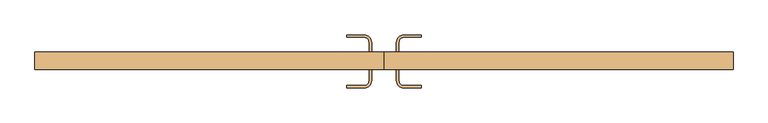
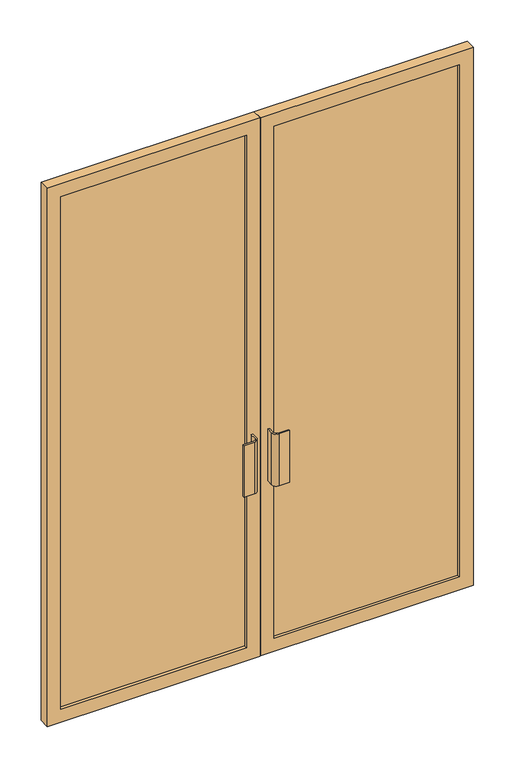
"""IFC4 building model written with IfcOpenShell, lengths in millimetres: door geometry, Porta-Parede-Cortina-Frente de loja-Dupla : Porta-Parede-Cortina-Frente de loja-Dupla."""

from ifc_helpers import new_model, si_unit, point, frame, frame_2d, origin, place, context, project, spatial, polyline, circle_curve, trimmed, segment, composite_curve, outline, extrude, source, transform, mapped, element, save


def door_024b7173(model_context):
    return source(origin(), model_context, "Body", "SweptSolid", [
        extrude(outline(polyline([(2375.0, 0.8168501), (0.0, 0.8168501), (0.0, 890.0), (2375.0, 890.0), (2375.0, 0.8168501)]), holes=[polyline([(2317.85, 57.9668501), (2317.85, 832.85), (57.15, 832.85), (57.15, 57.9668501), (2317.85, 57.9668501)])]), frame((0.0, 15.55, 0.0), z_axis=(0.0, 1.0, 0.0), x_axis=(0.0, 0.0, 1.0)), (0.0, 0.0, 1.0), 44.45),
        extrude(outline(polyline([(2375.0, -0.7706499), (2375.0, -890.0), (0.0, -890.0), (0.0, -0.7706499), (2375.0, -0.7706499)]), holes=[polyline([(2317.85, -832.85), (2317.85, -57.9206499), (57.15, -57.9206499), (57.15, -832.85), (2317.85, -832.85)])]), frame((0.0, 15.55, 0.0), z_axis=(0.0, 1.0, 0.0), x_axis=(0.0, 0.0, 1.0)), (0.0, 0.0, 1.0), 44.45),
        extrude(outline(polyline([(832.85, 28.25), (57.9668501, 28.25), (57.9668501, 47.3), (832.85, 47.3), (832.85, 28.25)])), frame((0.0, 0.0, 57.15), z_axis=(0.0, 0.0, 1.0), x_axis=(1.0, 0.0, 0.0)), (0.0, 0.0, 1.0), 2260.7),
        extrude(outline(polyline([(-57.9206499, 28.25), (-832.85, 28.25), (-832.85, 47.3), (-57.9206499, 47.3), (-57.9206499, 28.25)])), frame((0.0, 0.0, 57.15), z_axis=(0.0, 0.0, 1.0), x_axis=(1.0, 0.0, 0.0)), (0.0, 0.0, 1.0), 2260.7),
        extrude(outline(composite_curve([segment(trimmed(circle_curve(frame_2d((-50.7768999, -12.7)), 19.05), [point((-31.7268999, -12.7))], [point((-50.7768999, -31.75))], False, "CARTESIAN"), True, "CONTINUOUS"), segment(polyline([(-50.7768999, -31.75), (-95.2268999, -31.75), (-95.2268999, -25.4), (-50.7768999, -25.4)]), True, "CONTINUOUS"), segment(trimmed(circle_curve(frame_2d((-50.7768999, -12.7)), 12.7), [point((-50.7768999, -25.4))], [point((-38.0768999, -12.7))], True, "CARTESIAN"), True, "CONTINUOUS"), segment(polyline([(-38.0768999, -12.7), (-38.0768999, 15.55), (-31.7268999, 15.55), (-31.7268999, -12.7)]), True, "CONTINUOUS")], self_intersect=False)), frame((0.0, 0.0, 762.0), z_axis=(0.0, 0.0, 1.0), x_axis=(1.0, 0.0, 0.0)), (0.0, 0.0, 1.0), 228.6),
        extrude(outline(composite_curve([segment(polyline([(31.7731001, -12.7), (31.7731001, 15.55), (38.1231001, 15.55), (38.1231001, -12.7)]), True, "CONTINUOUS"), segment(trimmed(circle_curve(frame_2d((50.8231001, -12.7)), 12.7), [point((38.1231001, -12.7))], [point((50.8231001, -25.4))], True, "CARTESIAN"), True, "CONTINUOUS"), segment(polyline([(50.8231001, -25.4), (95.2731001, -25.4), (95.2731001, -31.75), (50.8231001, -31.75)]), True, "CONTINUOUS"), segment(trimmed(circle_curve(frame_2d((50.8231001, -12.7)), 19.05), [point((50.8231001, -31.75))], [point((31.7731001, -12.7))], False, "CARTESIAN"), True, "CONTINUOUS")], self_intersect=False)), frame((0.0, 0.0, 762.0), z_axis=(0.0, 0.0, 1.0), x_axis=(1.0, 0.0, 0.0)), (0.0, 0.0, 1.0), 228.6),
        extrude(outline(composite_curve([segment(polyline([(-31.7268999, 85.4), (-31.7268999, 60.0), (-38.0768999, 60.0), (-38.0768999, 85.4)]), True, "CONTINUOUS"), segment(trimmed(circle_curve(frame_2d((-50.7768999, 85.4)), 12.7), [point((-38.0768999, 85.4))], [point((-50.7768999, 98.1))], True, "CARTESIAN"), True, "CONTINUOUS"), segment(polyline([(-50.7768999, 98.1), (-95.2268999, 98.1), (-95.2268999, 104.45), (-50.7768999, 104.45)]), True, "CONTINUOUS"), segment(trimmed(circle_curve(frame_2d((-50.7768999, 85.4)), 19.05), [point((-50.7768999, 104.45))], [point((-31.7268999, 85.4))], False, "CARTESIAN"), True, "CONTINUOUS")], self_intersect=False)), frame((0.0, 0.0, 762.0), z_axis=(0.0, 0.0, 1.0), x_axis=(1.0, 0.0, 0.0)), (0.0, 0.0, 1.0), 228.6),
        extrude(outline(composite_curve([segment(trimmed(circle_curve(frame_2d((50.8231001, 85.4)), 19.05), [point((31.7731001, 85.4))], [point((50.8231001, 104.45))], False, "CARTESIAN"), True, "CONTINUOUS"), segment(polyline([(50.8231001, 104.45), (95.2731001, 104.45), (95.2731001, 98.1), (50.8231001, 98.1)]), True, "CONTINUOUS"), segment(trimmed(circle_curve(frame_2d((50.8231001, 85.4)), 12.7), [point((50.8231001, 98.1))], [point((38.1231001, 85.4))], True, "CARTESIAN"), True, "CONTINUOUS"), segment(polyline([(38.1231001, 85.4), (38.1231001, 60.0), (31.7731001, 60.0), (31.7731001, 85.4)]), True, "CONTINUOUS")], self_intersect=False)), frame((0.0, 0.0, 762.0), z_axis=(0.0, 0.0, 1.0), x_axis=(1.0, 0.0, 0.0)), (0.0, 0.0, 1.0), 228.6),
    ])


if __name__ == "__main__":
    model = new_model("IFC4")
    model_context = context("Model", 3, world=origin())
    ifc_project = project(units=[si_unit("LENGTHUNIT", "METRE", prefix="MILLI")], contexts=[model_context])
    site = spatial("IfcSite", under=ifc_project)
    building = spatial("IfcBuilding", under=site)
    placement = place(None, origin())
    door_shape = door_024b7173(model_context)
    element("IfcDoor", 1, ObjectType="Porta-Parede-Cortina-Frente de loja-Dupla : Porta-Parede-Cortina-Frente de loja-Dupla", at=placement, inside=building, context=model_context, shape_type="MappedRepresentation", body=[
        mapped(door_shape, transform((0.0, 0.0, 0.0), x_axis=(1.0, 0.0, 0.0), y_axis=(0.0, 1.0, 0.0), z_axis=(0.0, 0.0, 1.0))),
    ])
    save(model, "model.ifc")

# Revit data of these elements
# Type "Porta-Parede-Cortina-Frente de loja-Dupla : Porta-Parede-Cortina-Frente de loja-Dupla"
#   Type Mark = "40"
#   Construction Type Id = "opn-d46"
#   Assembly Code = "B2030100"
#   Analytic Construction = "Moldura de metal, porta de vidro duplo"
#   Largura [instance default] = 1.80 m
#   Thermal Resistance (R) = 0.242926 (m²·K)/W
#   Ângulo de abertura [instance default] = 90.00°
#   Largura do painel [instance default] = 0.90 m
#   Deslocamento = 0.06 m
#   Heat Transfer Coefficient (U) = 4.11674 W/(m²·K)
#   Function = 1
#   Material da moldura = Alumín. 1
#   Material da maçaneta = Alumín. 1
#   Vidraça = Vidro
#   Visual Light Transmittance = 0
#   Solar Heat Gain Coefficient = 0
# Element 1 (IfcDoor, "Porta-Parede-Cortina-Frente de loja-Dupla : Porta-Parede-Cortina-Frente de loja-Dupla")
#   Largura = 1.78 m
#   Largura do painel = 0.89 m
#   Materials on its faces: "Alumín. 1", "Vidro"
# Materials
#   "Alumín. 1": class "Metal", colour RGB 247 247 247, transparency 0, Description = "Alumín. 6061", Cost = 0
#   "Vidro": class "Vidro", colour RGB 0 128 192, transparency 0.9, Description = "Vidro de sílica", Cost = 0
